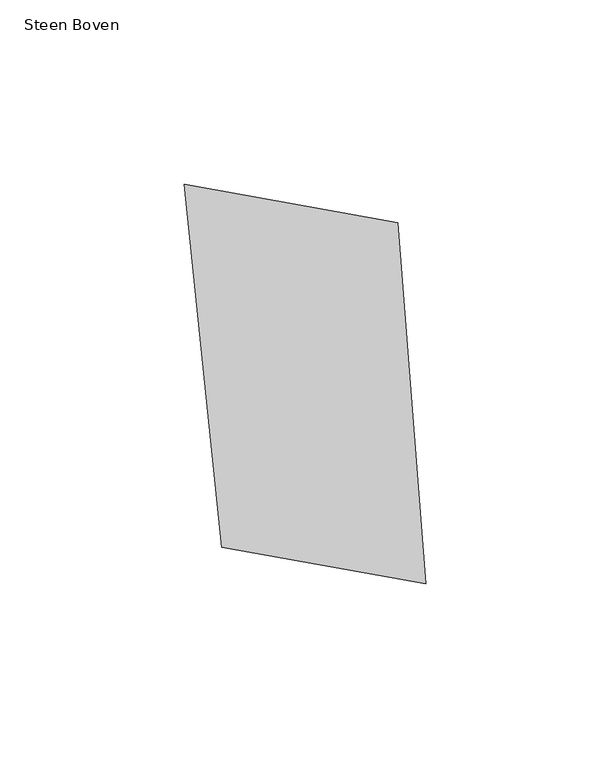
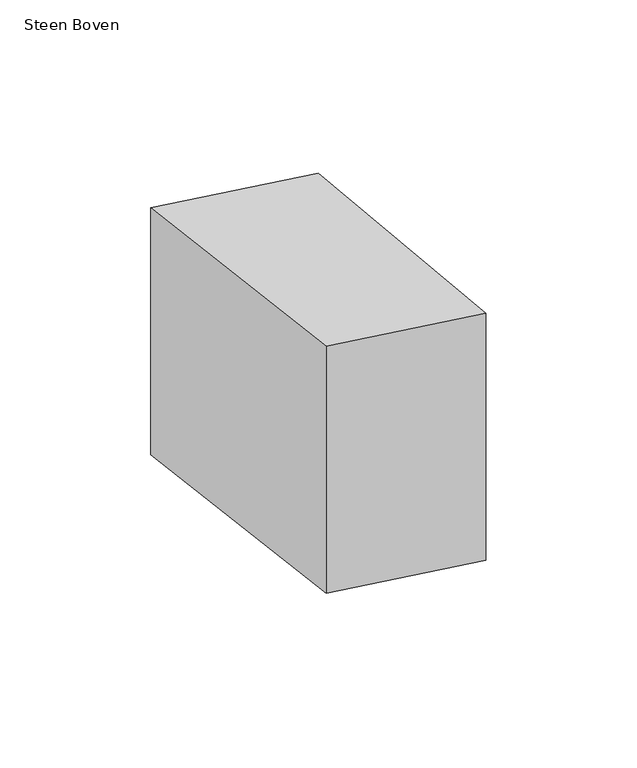
"""IFC4 building model written with IfcOpenShell, lengths in millimetres: proxy geometry, 00_GMA_steen_versie_4 : Steen Boven."""

from ifc_helpers import new_model, si_unit, origin, origin_with_axes, place, context, project, spatial, polyline, outline, extrude, source, transform, mapped, element, save


def steen_boven_00b99d4d(model_context):
    return source(origin(), model_context, "Body", "SweptSolid", [
        extrude(outline(polyline([(96.6422576, 121.0208269), (104.237318, 22.9349687), (48.8019465, 32.9369828), (38.6190863, 131.5205321), (96.6422576, 121.0208269)])), origin_with_axes(), (0.0, 0.0, 1.0), 100.0),
    ])


if __name__ == "__main__":
    model = new_model("IFC4")
    model_context = context("Model", 3, world=origin())
    ifc_project = project(units=[si_unit("LENGTHUNIT", "METRE", prefix="MILLI")], contexts=[model_context])
    site = spatial("IfcSite", under=ifc_project)
    building = spatial("IfcBuilding", under=site)
    placement = place(None, origin())
    steen_boven_shape = steen_boven_00b99d4d(model_context)
    element("IfcBuildingElementProxy", 1, Name="00_GMA_steen_versie_4 : Steen Boven", ObjectType="00_GMA_steen_versie_4 : Steen Boven", at=placement, inside=building, context=model_context, shape_type="MappedRepresentation", body=[
        mapped(steen_boven_shape, transform((0.0, 0.0, 0.0), x_axis=(1.0, 0.0, 0.0), y_axis=(0.0, 1.0, 0.0), z_axis=(0.0, 0.0, 1.0))),
    ])
    save(model, "model.ifc")

# Revit data of these elements
# Type "00_GMA_steen_versie_4 : Steen Boven"
#   StootVoegHalfBoven [instance default] = 5 mm
#   StootVoegHalf [instance default] = 5 mm
#   StootVoegBreedteOnder = 10 mm
#   StootVoegBreedteBoven = 10 mm
#   Steendikte = 100 mm
#   LintVoegOnderHalf = 5 mm
#   LintVoegOnder = 10 mm
#   LintVoegBovenHalf = 0 mm
#   LintVoegBoven = 0 mm
#   materiaal = none
#   MateriaalVoeg = none
#   Default Elevation = 0
